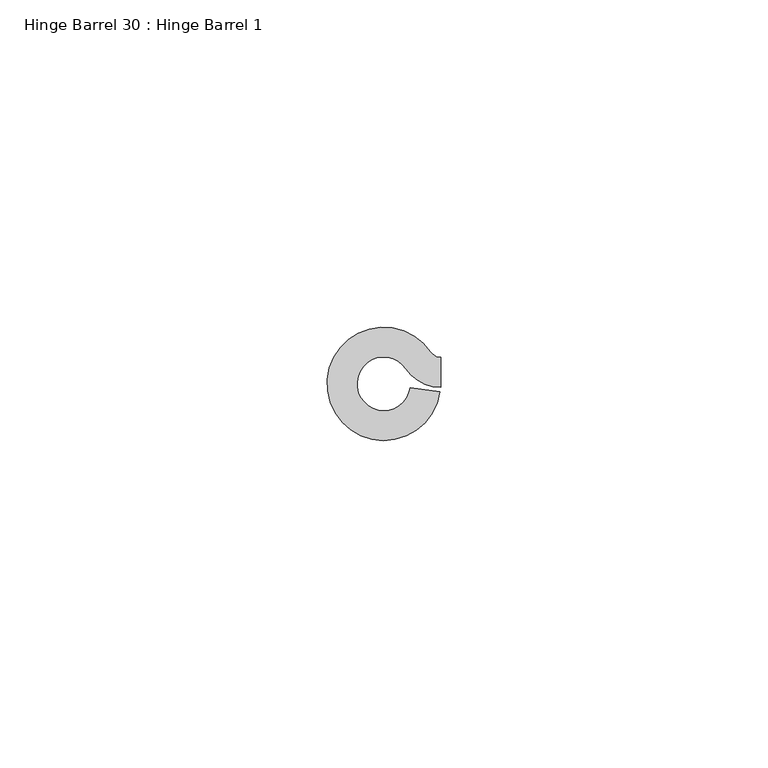
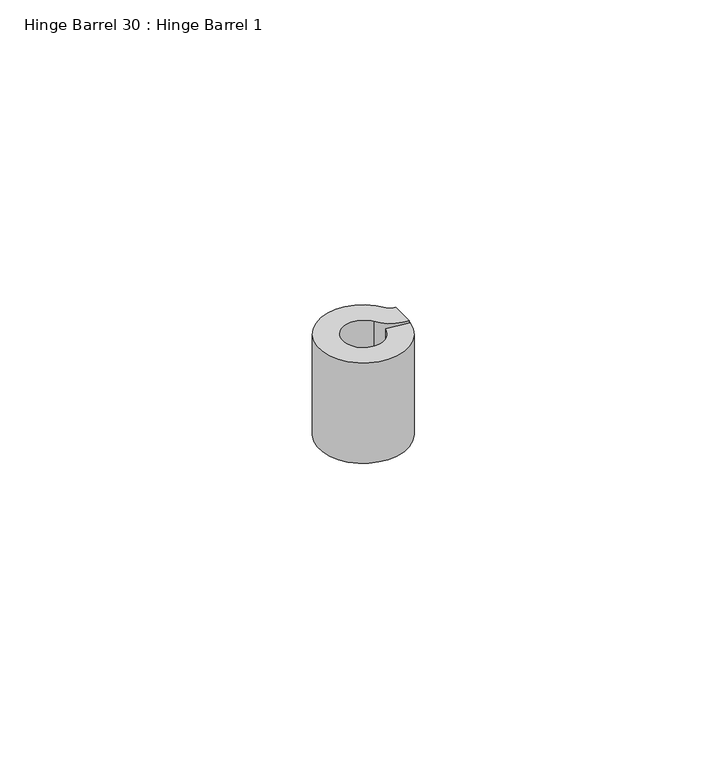
"""IFC4 building model written with IfcOpenShell, lengths in millimetres: proxy geometry, Hinge Barrel 30 : Hinge Barrel 1."""

from ifc_helpers import new_model, si_unit, point, frame, frame_2d, origin, place, context, project, spatial, polyline, circle_curve, trimmed, segment, composite_curve, outline, extrude, source, transform, mapped, element, save


def hinge_barrel_30_hinge_barrel_1_18e6ea9c(model_context):
    return source(origin(), model_context, "Body", "SweptSolid", [
        extrude(outline(composite_curve([segment(trimmed(circle_curve(frame_2d((587319.1320739, -531776.6049841)), 4.0894), [point((587322.5194669, -531774.3139665))], [point((587323.1821338, -531777.1708529))], True, "CARTESIAN"), True, "CONTINUOUS"), segment(polyline([(587323.1821338, -531777.1708529), (587327.7022899, -531777.8024028)]), True, "CONTINUOUS"), segment(trimmed(circle_curve(frame_2d((587319.1320739, -531776.6049841)), 8.6534625), [point((587327.7022899, -531777.8024028))], [point((587326.3000393, -531771.7570273))], False, "CARTESIAN"), True, "CONTINUOUS"), segment(trimmed(circle_curve(frame_2d((587327.8245257, -531770.7259615)), 1.8404226), [point((587326.3000393, -531771.7570273))], [point((587327.8245257, -531772.5663841))], True, "CARTESIAN"), True, "CONTINUOUS"), segment(polyline([(587327.8245257, -531772.5663841), (587327.8245257, -531777.1304466)]), True, "CONTINUOUS"), segment(trimmed(circle_curve(frame_2d((587327.8245257, -531770.7259615)), 6.4044851), [point((587327.8245257, -531777.1304466))], [point((587322.5194669, -531774.3139665))], False, "CARTESIAN"), True, "CONTINUOUS")], self_intersect=False)), frame((0.0, 0.0, 1250.95), z_axis=(0.0, 0.0, 1.0), x_axis=(1.0, 0.0, 0.0)), (0.0, 0.0, 1.0), 20.8359375),
    ])


if __name__ == "__main__":
    model = new_model("IFC4")
    model_context = context("Model", 3, world=origin())
    ifc_project = project(units=[si_unit("LENGTHUNIT", "METRE", prefix="MILLI")], contexts=[model_context])
    site = spatial("IfcSite", under=ifc_project)
    building = spatial("IfcBuilding", under=site)
    placement = place(None, origin())
    hinge_barrel_30_hinge_barrel_1_shape = hinge_barrel_30_hinge_barrel_1_18e6ea9c(model_context)
    element("IfcBuildingElementProxy", 1, Name="Hinge Barrel 30 : Hinge Barrel 1", ObjectType="Hinge Barrel 30 : Hinge Barrel 1", at=placement, inside=building, context=model_context, shape_type="MappedRepresentation", body=[
        mapped(hinge_barrel_30_hinge_barrel_1_shape, transform((0.0, 0.0, 0.0), x_axis=(1.0, 0.0, 0.0), y_axis=(0.0, 1.0, 0.0), z_axis=(0.0, 0.0, 1.0))),
    ])
    save(model, "model.ifc")

# Revit data of these elements
# Element 1 (IfcBuildingElementProxy, "Hinge Barrel 30 : Hinge Barrel 1")
#   Materials on its faces: "6\"X6\" WELD-ON STL BUTT HINGE"
# Materials
#   "6\"X6\" WELD-ON STL BUTT HINGE": class "Metal", colour RGB 189 187 185, transparency 0, Description = "Carbon steel", Cost = 0
